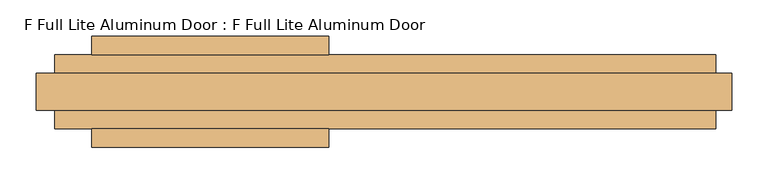
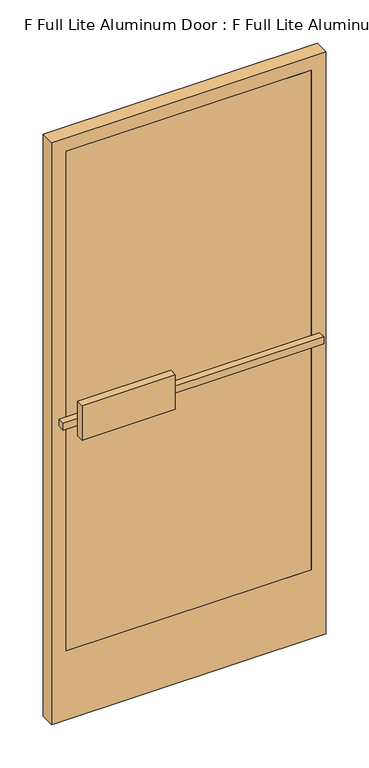
"""IFC4 building model written with IfcOpenShell, lengths in millimetres: door geometry, F Full Lite Aluminum Door : F Full Lite Aluminum Door."""

from ifc_helpers import new_model, si_unit, frame, origin, place, context, project, spatial, polyline, outline, extrude, source, transform, mapped, element, save


def f_full_lite_aluminum_door_f_full_lite_aluminum_door_afe42425(model_context):
    return source(origin(), model_context, "Body", "SweptSolid", [
        extrude(outline(polyline([(427.434375, 0.0), (427.434375, -50.8), (-427.434375, -50.8), (-427.434375, 0.0), (427.434375, 0.0)])), frame((0.0, 0.0, 254.0), z_axis=(0.0, 0.0, 1.0), x_axis=(1.0, 0.0, 0.0)), (0.0, 0.0, 1.0), 1840.70625),
        extrude(outline(polyline([(2145.50625, -478.234375), (0.0, -478.234375), (0.0, 478.234375), (2145.50625, 478.234375), (2145.50625, -478.234375)]), holes=[polyline([(2094.70625, -427.434375), (2094.70625, 427.434375), (254.0, 427.434375), (254.0, -427.434375), (2094.70625, -427.434375)])]), frame((0.0, -50.8, 0.0), z_axis=(0.0, 1.0, 0.0), x_axis=(0.0, 0.0, 1.0)), (0.0, 0.0, 1.0), 50.8),
        extrude(outline(polyline([(-402.034375, 25.4), (-402.034375, 50.8), (-76.2, 50.8), (-76.2, 25.4), (-402.034375, 25.4)])), frame((0.0, 0.0, 1041.4), z_axis=(0.0, 0.0, 1.0), x_axis=(1.0, 0.0, 0.0)), (0.0, 0.0, 1.0), 127.0),
        extrude(outline(polyline([(-76.2, -76.2), (-76.2, -101.6), (-402.034375, -101.6), (-402.034375, -76.2), (-76.2, -76.2)])), frame((0.0, 0.0, 1053.30625), z_axis=(0.0, 0.0, 1.0), x_axis=(1.0, 0.0, 0.0)), (0.0, 0.0, 1.0), 127.0),
        extrude(outline(polyline([(-452.834375, 0.0), (-452.834375, 25.4), (456.4629464, 25.4), (456.4629464, 0.0), (-452.834375, 0.0)])), frame((0.0, 0.0, 1104.10625), z_axis=(0.0, 0.0, 1.0), x_axis=(1.0, 0.0, 0.0)), (0.0, 0.0, 1.0), 25.4),
        extrude(outline(polyline([(456.4629464, -50.8), (456.4629464, -76.2), (-452.834375, -76.2), (-452.834375, -50.8), (456.4629464, -50.8)])), frame((0.0, 0.0, 1092.2), z_axis=(0.0, 0.0, 1.0), x_axis=(1.0, 0.0, 0.0)), (0.0, 0.0, 1.0), 25.4),
    ])


if __name__ == "__main__":
    model = new_model("IFC4")
    model_context = context("Model", 3, world=origin())
    ifc_project = project(units=[si_unit("LENGTHUNIT", "METRE", prefix="MILLI")], contexts=[model_context])
    site = spatial("IfcSite", under=ifc_project)
    building = spatial("IfcBuilding", under=site)
    placement = place(None, origin())
    f_full_lite_aluminum_door_f_full_lite_aluminum_door_shape = f_full_lite_aluminum_door_f_full_lite_aluminum_door_afe42425(model_context)
    element("IfcDoor", 1, ObjectType="F Full Lite Aluminum Door : F Full Lite Aluminum Door", at=placement, inside=building, context=model_context, shape_type="MappedRepresentation", body=[
        mapped(f_full_lite_aluminum_door_f_full_lite_aluminum_door_shape, transform((0.0, 0.0, 0.0), x_axis=(1.0, 0.0, 0.0), y_axis=(0.0, 1.0, 0.0), z_axis=(0.0, 0.0, 1.0))),
    ])
    save(model, "model.ifc")

# Revit data of these elements
# Type "F Full Lite Aluminum Door : F Full Lite Aluminum Door"
#   Type Mark = "20"
#   Construction Type Id = "SGL"
#   Assembly Code = "B2030100"
#   Analytic Construction = "Large single-glazed windows"
#   Visual Light Transmittance = 0.9
#   Thermal Resistance (R) = 0.179801 (m²·K)/W
#   Solar Heat Gain Coefficient = 0.86
#   Heat Transfer Coefficient (U) = 5.5617 W/(m²·K)
#   Offset = 0' - 2"
#   Function = 1
#   Handle Material = Aluminum
#   Glazing Material = Glass
# Element 1 (IfcDoor, "F Full Lite Aluminum Door : F Full Lite Aluminum Door")
#   Materials on its faces: "Aluminum", "Glass"
# Materials
#   "Aluminum": class "Metal", colour RGB 247 247 247, transparency 0, Description = "Aluminum 6061", Cost = 0
#   "Glass": class "Unassigned", colour RGB 0 0 255, transparency 0.75
